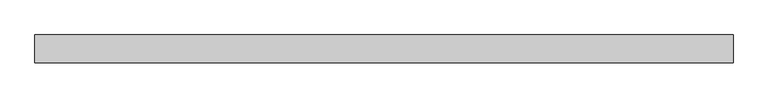
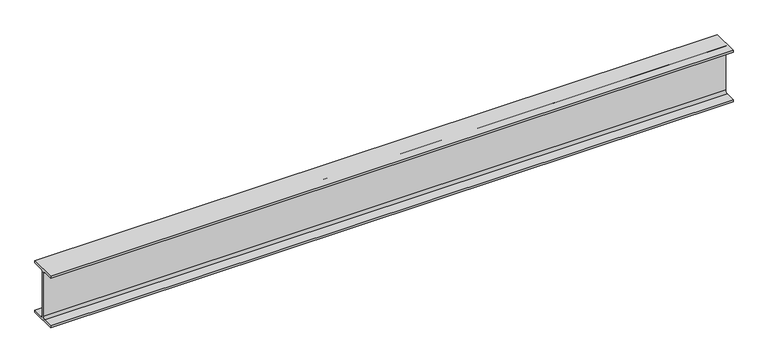
"""IFC4 building model written with IfcOpenShell, lengths in millimetres: beam geometry, 0912_Steel Framing_H-KSD3502 : H_SB_ASB_H-250x125x6x9."""

from ifc_helpers import new_model, si_unit, point, frame, frame_2d, origin, place, context, project, spatial, polyline, circle_curve, trimmed, segment, composite_curve, outline, extrude, source, transform, mapped, element, save


def beam_d1df00b5(model_context):
    return source(origin(), model_context, "Body", "SweptSolid", [
        extrude(outline(composite_curve([segment(polyline([(62.5, -116.0), (62.5, -125.0), (-62.5, -125.0), (-62.5, -116.0), (-15.0, -116.0)]), True, "CONTINUOUS"), segment(trimmed(circle_curve(frame_2d((-15.0, -104.0)), 12.0), [point((-15.0, -116.0))], [point((-3.0, -104.0))], True, "CARTESIAN"), True, "CONTINUOUS"), segment(polyline([(-3.0, -104.0), (-3.0, 104.0)]), True, "CONTINUOUS"), segment(trimmed(circle_curve(frame_2d((-15.0, 104.0)), 12.0), [point((-3.0, 104.0))], [point((-15.0, 116.0))], True, "CARTESIAN"), True, "CONTINUOUS"), segment(polyline([(-15.0, 116.0), (-62.5, 116.0), (-62.5, 125.0), (62.5, 125.0), (62.5, 116.0), (15.0, 116.0)]), True, "CONTINUOUS"), segment(trimmed(circle_curve(frame_2d((15.0, 104.0)), 12.0), [point((15.0, 116.0))], [point((3.0, 104.0))], True, "CARTESIAN"), True, "CONTINUOUS"), segment(polyline([(3.0, 104.0), (3.0, -104.0)]), True, "CONTINUOUS"), segment(trimmed(circle_curve(frame_2d((15.0, -104.0)), 12.0), [point((3.0, -104.0))], [point((15.0, -116.0))], True, "CARTESIAN"), True, "CONTINUOUS"), segment(polyline([(15.0, -116.0), (62.5, -116.0)]), True, "CONTINUOUS")], self_intersect=False)), frame((-1654.8, 0.0, 0.0), z_axis=(1.0, 0.0, 0.0), x_axis=(0.0, 1.0, 0.0)), (0.0, 0.0, 1.0), 3149.3360727),
    ])


if __name__ == "__main__":
    model = new_model("IFC4")
    model_context = context("Model", 3, world=origin())
    ifc_project = project(units=[si_unit("LENGTHUNIT", "METRE", prefix="MILLI")], contexts=[model_context])
    site = spatial("IfcSite", under=ifc_project)
    building = spatial("IfcBuilding", under=site)
    placement = place(None, origin())
    beam_shape = beam_d1df00b5(model_context)
    element("IfcBeam", 1, ObjectType="0912_Steel Framing_H-KSD3502 : H_SB_ASB_H-250x125x6x9", at=placement, inside=building, context=model_context, shape_type="MappedRepresentation", body=[
        mapped(beam_shape, transform((0.0, 0.0, 0.0), x_axis=(1.0, 0.0, 0.0), y_axis=(0.0, 1.0, 0.0), z_axis=(0.0, 0.0, 1.0))),
    ])
    save(model, "model.ifc")

# Revit data of these elements
# Type "0912_Steel Framing_H-KSD3502 : H_SB_ASB_H-250x125x6x9"
#   H_WM Code_1 = "S01AA003-00001 | Main Steel Structure Fabrication Work | Shelter/Building | Light Steel - Standard (30KG/M>Weight) | Material: (   )"
#   H_WM Code_2 = "S03AA029-00001 | Main Steel Structure Erection Work | Shelter/Building | Light Steel (30KG/M>Weight) | Material: (   )"
#   H_WM Code_3 = "S01AA010-00001 | Main Steel Structure Fabrication Work | Shelter/Building | Steel Painting/Coating | for Non-Fireproofed Steel Surface, Surface Preparation, Primer, Second & Final Coat | Material: (   )"
#   H_Q'ty Cal Type Tag = "SB-Q2"
#   Width = 12.5 cm
#   Web Thickness = 0.6 cm
#   Web Fillet = 1.2 cm
#   Warping Constant = 42539.8 cm⁶
#   W = 0
#   Torsional Moment of Inertia = 7.8102 cm⁴
#   Section Area = 37.66 cm²
#   Plastic Modulus weak axis = 73.1 cm³
#   Plastic Modulus strong axis = 366.0 cm³
#   Perimeter = 0.97 m²/m
#   Nominal Weight = 29.60 kgf/m
#   Moment of Inertia weak axis = 294.00 cm⁴
#   Moment of Inertia strong axis = 4050.00 cm⁴
#   Height = 25.0 cm
#   Flange Thickness = 0.9 cm
#   Elastic Modulus weak axis = 47.0 cm³
#   Elastic Modulus strong axis = 324.0 cm³
#   Centroid Vertical = 12.5 cm
#   Centroid Horizontal = 6.25 cm
#   Ix = 40500000
#   Length [instance default] = 1.5240 m
#   Zx = 366000
#   b = 0.1250 m
#   h = 0.2500 m
#   r = 0.0120 m
#   s = 0.0060 m
#   t = 0.0090 m
#   A = 0.003766 m²
#   Structural Material [instance default] = Steel, 45-345
#   Assembly Code = ""
# Element 1 (IfcBeam, "0912_Steel Framing_H-KSD3502 : H_SB_ASB_H-250x125x6x9")
#   Structural Material = none
# Materials
#   "Steel, 45-345": class "Metal", colour RGB 189 187 185, transparency 0, Description = "Steel 345 MPa", Cost = 0
